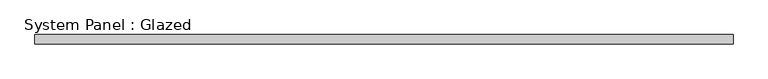
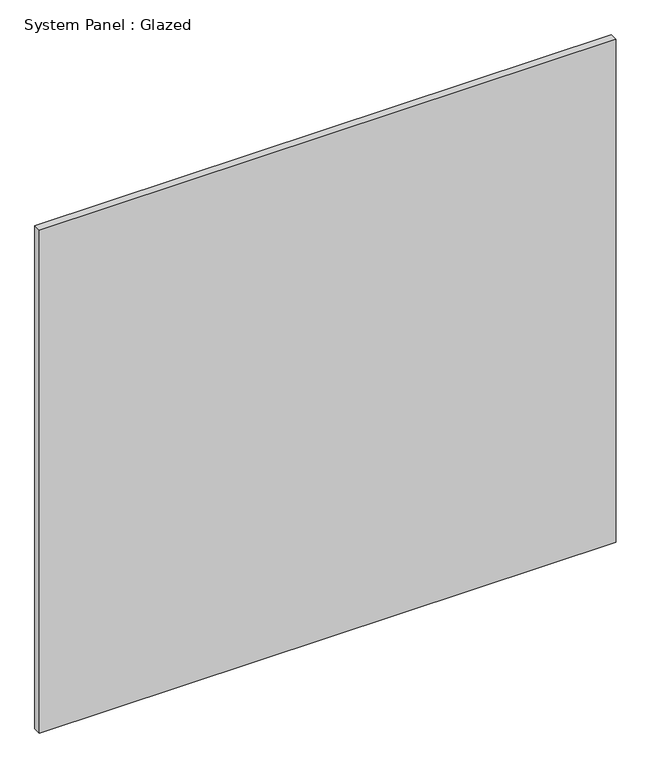
"""IFC4 building model written with IfcOpenShell, lengths in millimetres: plate geometry, System Panel : Glazed."""

from ifc_helpers import new_model, si_unit, origin, origin_with_axes, place, context, project, spatial, polyline, outline, extrude, source, transform, mapped, element, save


def system_panel_glazed_eda6632c(model_context):
    return source(origin(), model_context, "Body", "SweptSolid", [
        extrude(outline(polyline([(915.0000002, 24.5), (-915.0000002, 24.5), (-915.0000002, 49.5), (915.0000002, 49.5), (915.0000002, 24.5)])), origin_with_axes(), (0.0, 0.0, 1.0), 1686.2355347),
    ])


if __name__ == "__main__":
    model = new_model("IFC4")
    model_context = context("Model", 3, world=origin())
    ifc_project = project(units=[si_unit("LENGTHUNIT", "METRE", prefix="MILLI")], contexts=[model_context])
    site = spatial("IfcSite", under=ifc_project)
    building = spatial("IfcBuilding", under=site)
    placement = place(None, origin())
    system_panel_glazed_shape = system_panel_glazed_eda6632c(model_context)
    element("IfcPlate", 1, ObjectType="System Panel : Glazed", at=placement, inside=building, context=model_context, shape_type="MappedRepresentation", body=[
        mapped(system_panel_glazed_shape, transform((0.0, 0.0, 0.0), x_axis=(1.0, 0.0, 0.0), y_axis=(0.0, 1.0, 0.0), z_axis=(0.0, 0.0, 1.0))),
    ])
    save(model, "model.ifc")

# Revit data of these elements
# Element 1 (IfcPlate, "System Panel : Glazed")
#   Materials on its faces: "Glass"
# Materials
#   "Glass": class "Glass", colour RGB 218 227 224, transparency 0.85, Description = "Soda Lime Glass", Cost = 0
